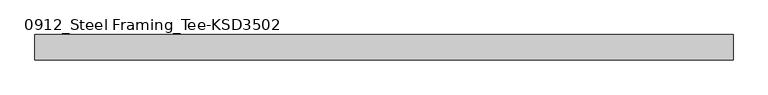
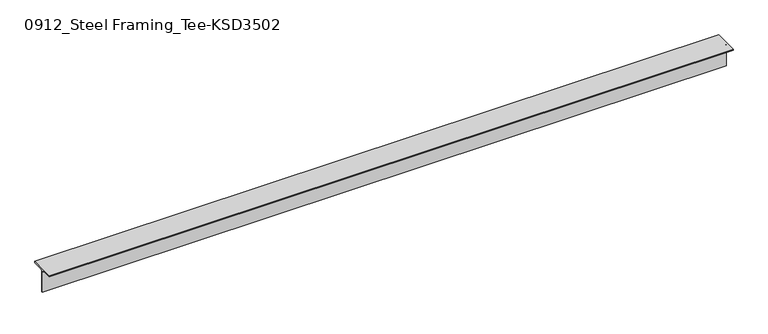
"""IFC4 building model written with IfcOpenShell, lengths in millimetres: member geometry, 0912_Steel Framing_Tee-KSD3502 : H_SB_ASB_CT-150x150x6.5x9."""

from ifc_helpers import new_model, si_unit, point, frame, frame_2d, origin, place, context, project, spatial, polyline, circle_curve, trimmed, segment, composite_curve, outline, extrude, source, transform, mapped, element, save


def member_0912_steel_framing_tee_ksd3502_428d2e16(model_context):
    return source(origin(), model_context, "Body", "SweptSolid", [
        extrude(outline(composite_curve([segment(polyline([(-75.0, 75.0), (75.0, 75.0), (75.0, 66.0), (16.25, 66.0)]), True, "CONTINUOUS"), segment(trimmed(circle_curve(frame_2d((16.25, 53.0)), 13.0), [point((16.25, 66.0))], [point((3.25, 53.0))], True, "CARTESIAN"), True, "CONTINUOUS"), segment(polyline([(3.25, 53.0), (3.25, -75.0), (-3.25, -75.0), (-3.25, 53.0)]), True, "CONTINUOUS"), segment(trimmed(circle_curve(frame_2d((-16.25, 53.0)), 13.0), [point((-3.25, 53.0))], [point((-16.25, 66.0))], True, "CARTESIAN"), True, "CONTINUOUS"), segment(polyline([(-16.25, 66.0), (-75.0, 66.0), (-75.0, 75.0)]), True, "CONTINUOUS")], self_intersect=False)), frame((-2046.05, 0.0, 0.0), z_axis=(1.0, 0.0, 0.0), x_axis=(0.0, 1.0, 0.0)), (0.0, 0.0, 1.0), 4152.3),
    ])


if __name__ == "__main__":
    model = new_model("IFC4")
    model_context = context("Model", 3, world=origin())
    ifc_project = project(units=[si_unit("LENGTHUNIT", "METRE", prefix="MILLI")], contexts=[model_context])
    site = spatial("IfcSite", under=ifc_project)
    building = spatial("IfcBuilding", under=site)
    placement = place(None, origin())
    member_0912_steel_framing_tee_ksd3502_shape = member_0912_steel_framing_tee_ksd3502_428d2e16(model_context)
    element("IfcMember", 1, ObjectType="0912_Steel Framing_Tee-KSD3502 : H_SB_ASB_CT-150x150x6.5x9", at=placement, inside=building, context=model_context, shape_type="MappedRepresentation", body=[
        mapped(member_0912_steel_framing_tee_ksd3502_shape, transform((0.0, 0.0, 0.0), x_axis=(1.0, 0.0, 0.0), y_axis=(0.0, 1.0, 0.0), z_axis=(0.0, 0.0, 1.0))),
    ])
    save(model, "model.ifc")

# Revit data of these elements
# Type "0912_Steel Framing_Tee-KSD3502 : H_SB_ASB_CT-150x150x6.5x9"
#   H_WM Code_1 = "S01AA003-00001 | Main Steel Structure Fabrication Work | Shelter/Building | Light Steel - Standard (30KG/M>Weight) | Material: (   )"
#   H_WM Code_2 = "S03AA029-00001 | Main Steel Structure Erection Work | Shelter/Building | Light Steel (30KG/M>Weight) | Material: (   )"
#   H_WM Code_3 = "S01AA010-00001 | Main Steel Structure Fabrication Work | Shelter/Building | Steel Painting/Coating | for Non-Fireproofed Steel Surface, Surface Preparation, Primer, Second & Final Coat | Material: (   )"
#   H_Q'ty Cal Type Tag = "SB-Q2"
#   Width = 15.0 cm
#   Web Thickness = 0.65 cm
#   Web Fillet = 1.3 cm
#   Section Area = 23.39 cm²
#   Perimeter = 0.60 m²/m
#   Nominal Weight = 18.40 kgf/m
#   Height = 15.0 cm
#   Flange Thickness = 0.9 cm
#   Centroid Vertical = 7.5 cm
#   Centroid Horizontal = 7.5 cm
#   Length [instance default] = 1.5000 m
#   Structural Material [instance default] = Steel, 45-345
#   Warping Constant = (empty or 0)
#   Torsional Moment of Inertia = 0
#   Section Name Key = ""
#   Plastic Modulus weak axis = 0
#   Plastic Modulus strong axis = 0
#   Moment of Inertia weak axis = 0
#   Moment of Inertia strong axis = 0
#   Elastic Modulus weak axis = 0
#   Elastic Modulus strong axis = 0
#   Bolt Spacing = 0
#   Assembly Code = ""
# Element 1 (IfcMember, "0912_Steel Framing_Tee-KSD3502 : H_SB_ASB_CT-150x150x6.5x9")
#   Structural Material = none
# Materials
#   "Steel, 45-345": class "Metal", colour RGB 189 187 185, transparency 0, Description = "Steel 345 MPa", Cost = 0
